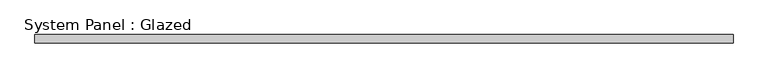
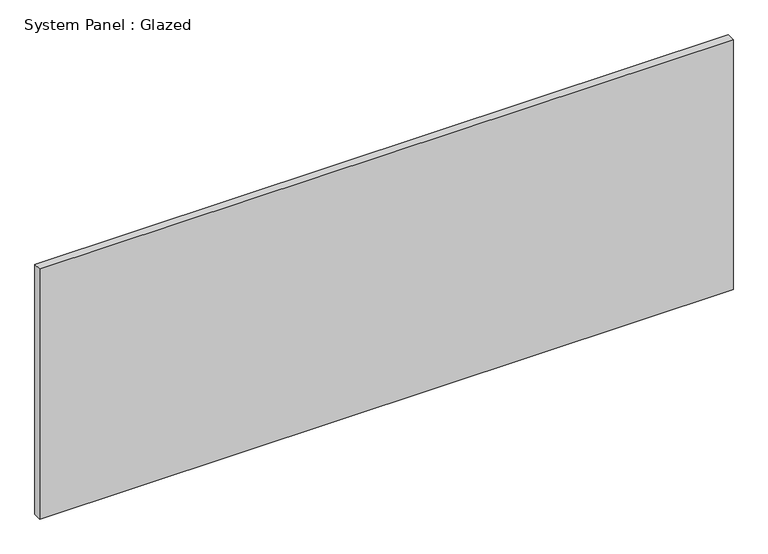
"""IFC4 building model written with IfcOpenShell, lengths in millimetres: plate geometry, System Panel : Glazed."""

from ifc_helpers import new_model, si_unit, origin, origin_with_axes, place, context, project, spatial, polyline, outline, extrude, source, transform, mapped, element, save


def system_panel_glazed_ad6e6b44(model_context):
    return source(origin(), model_context, "Body", "SweptSolid", [
        extrude(outline(polyline([(1073.15, -44.45), (-1073.15, -44.45), (-1073.15, -19.05), (1073.15, -19.05), (1073.15, -44.45)])), origin_with_axes(), (0.0, 0.0, 1.0), 819.15),
    ])


if __name__ == "__main__":
    model = new_model("IFC4")
    model_context = context("Model", 3, world=origin())
    ifc_project = project(units=[si_unit("LENGTHUNIT", "METRE", prefix="MILLI")], contexts=[model_context])
    site = spatial("IfcSite", under=ifc_project)
    building = spatial("IfcBuilding", under=site)
    placement = place(None, origin())
    system_panel_glazed_shape = system_panel_glazed_ad6e6b44(model_context)
    element("IfcPlate", 1, ObjectType="System Panel : Glazed", at=placement, inside=building, context=model_context, shape_type="MappedRepresentation", body=[
        mapped(system_panel_glazed_shape, transform((0.0, 0.0, 0.0), x_axis=(1.0, 0.0, 0.0), y_axis=(0.0, 1.0, 0.0), z_axis=(0.0, 0.0, 1.0))),
    ])
    save(model, "model.ifc")

# Revit data of these elements
# Type "System Panel : Glazed"
#   Construction Type Id = "GSP4R"
#   Analytic Construction = "1/8 in Pilkington single glazing"
#   Visual Light Transmittance = 0.9
#   Solar Heat Gain Coefficient = 0.86
#   Heat Transfer Coefficient (U) = 1.18115 BTU/(h·ft²·°F)
#   Define Thermal Properties by = 1
# Element 1 (IfcPlate, "System Panel : Glazed")
#   Materials on its faces: "Glass"
# Materials
#   "Glass": class "Glass", colour RGB 0 128 192, transparency 0.75, Description = "Soda Lime Glass", Cost = 0
